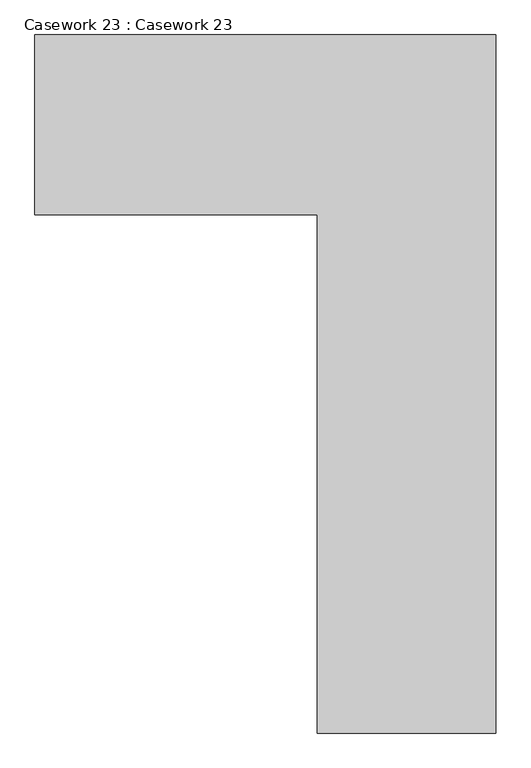
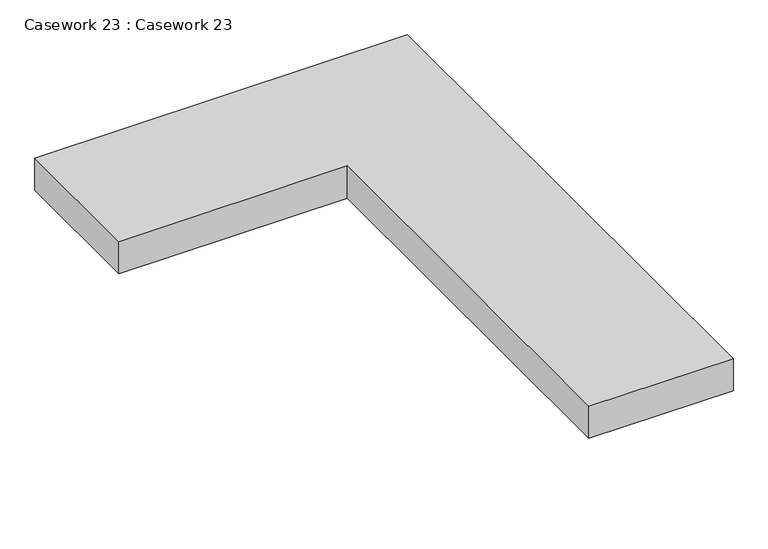
"""IFC4 building model written with IfcOpenShell, lengths in millimetres: furniture geometry, Casework 23 : Casework 23."""

from ifc_helpers import new_model, si_unit, frame, origin, place, context, project, spatial, polyline, outline, extrude, source, transform, mapped, element, save


def casework_23_casework_23_2977f71f(model_context):
    return source(origin(), model_context, "Body", "SweptSolid", [
        extrude(outline(polyline([(-34337.4785979, 275082.839438), (-35636.855403, 275082.839438), (-35636.855403, 278859.6613827), (-37694.2539888, 278859.6613827), (-37694.2539888, 280169.3737113), (-34337.4785979, 280169.3737113), (-34337.4785979, 275082.839438)])), frame((0.0, 0.0, 3048.0), z_axis=(0.0, 0.0, 1.0), x_axis=(1.0, 0.0, 0.0)), (0.0, 0.0, 1.0), 305.2489812),
    ])


if __name__ == "__main__":
    model = new_model("IFC4")
    model_context = context("Model", 3, world=origin())
    ifc_project = project(units=[si_unit("LENGTHUNIT", "METRE", prefix="MILLI")], contexts=[model_context])
    site = spatial("IfcSite", under=ifc_project)
    building = spatial("IfcBuilding", under=site)
    placement = place(None, origin())
    casework_23_casework_23_shape = casework_23_casework_23_2977f71f(model_context)
    element("IfcFurniture", 1, ObjectType="Casework 23 : Casework 23", at=placement, inside=building, context=model_context, shape_type="MappedRepresentation", body=[
        mapped(casework_23_casework_23_shape, transform((0.0, 0.0, 0.0), x_axis=(1.0, 0.0, 0.0), y_axis=(0.0, 1.0, 0.0), z_axis=(0.0, 0.0, 1.0))),
    ])
    save(model, "model.ifc")

# Revit data of these elements
# Element 1 (IfcFurniture, "Casework 23 : Casework 23")
#   Materials on its faces: "PAINTED STEEL C CHANNEL"
# Materials
#   "PAINTED STEEL C CHANNEL": class "Generic", colour RGB 88 62 61, transparency 0, Cost = 0
